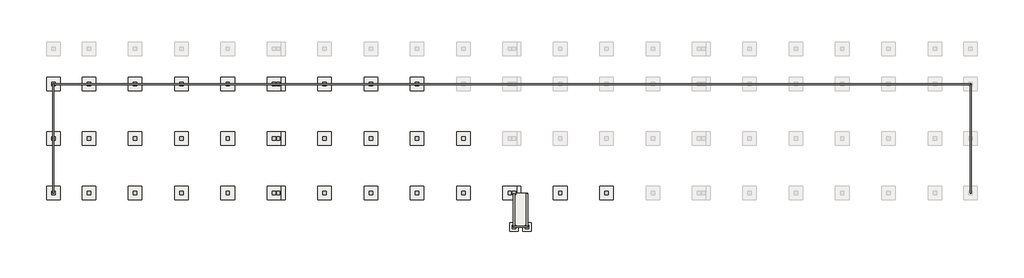
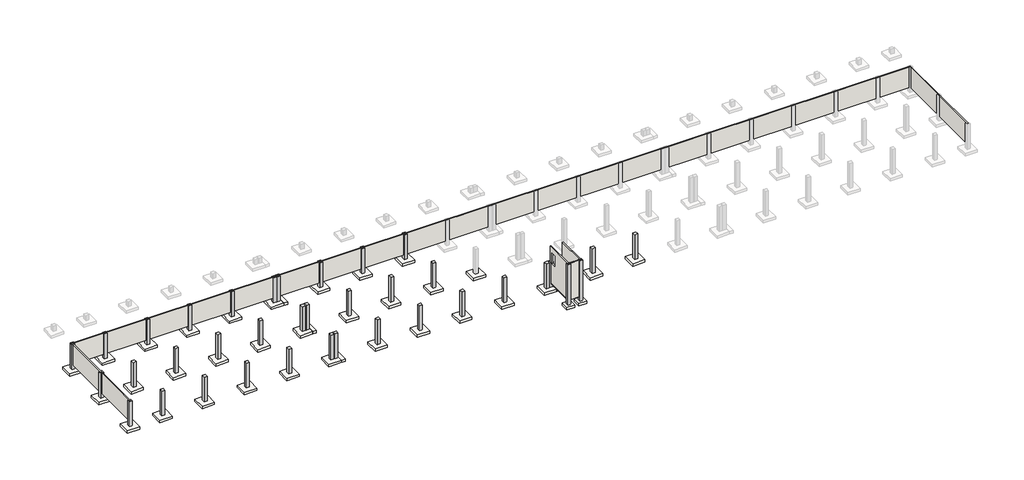
# Not in any storey, part 1 of 3: 39 slabs, 37 columns, 6 walls.
"""IFC4 building model written with IfcOpenShell, lengths in millimetres."""

import ifcopenshell
import ifcopenshell.guid

model = None  # the IFC model being written
_history = None  # IfcOwnerHistory: only IFC2X3 demands one
_inside = {}  # id of a spatial element -> (the spatial element, [elements in it])
_under = {}  # id of a project, library or spatial element -> (it, [spatial elements below it])
_declared = {}  # id of a project -> (the project, [libraries it declares])
_typed = {}  # id of a type object -> (the type object, [elements of that type])
_made_of = {}  # id of a material, layer set ... -> (it, [elements and type objects made of it])


def new_model(schema):
    """Start an empty IFC model of exactly this schema.

    Asked for "IFC4X3", IfcOpenShell would pick the latest addendum, in which some entities
    have other attributes; the version numbers below select the first issue.
    IFC2X3 requires an IfcOwnerHistory on every rooted entity: one is made here for all.
    """
    global model, _history
    if schema == "IFC4X3":
        model = ifcopenshell.file(schema_version=(4, 3, 0, 0))
    else:
        model = ifcopenshell.file(schema=schema)
    _inside.clear()
    _under.clear()
    _declared.clear()
    _typed.clear()
    _made_of.clear()
    _history = None
    if model.schema == "IFC2X3":
        org = make("IfcOrganization", Name="unknown")
        user = make(
            "IfcPersonAndOrganization",
            ThePerson=make("IfcPerson", FamilyName="unknown"),
            TheOrganization=org,
        )
        app = make(
            "IfcApplication",
            ApplicationDeveloper=org,
            Version="unknown",
            ApplicationFullName="unknown",
            ApplicationIdentifier="unknown",
        )
        _history = make(
            "IfcOwnerHistory",
            OwningUser=user,
            OwningApplication=app,
            ChangeAction="ADDED",
            CreationDate=0,
        )
    return model


def make(cls, **values):
    """One entity of the class cls with the attributes given. An attribute that is None is left unset."""
    return model.create_entity(
        cls, **{name: value for name, value in values.items() if value is not None}
    )


def rooted(cls, **values):
    """An entity with a GlobalId (a new one), such as an element, a storey or a relation."""
    return make(cls, GlobalId=ifcopenshell.guid.new(), OwnerHistory=_history, **values)


def si_unit(unit_type, name, prefix=None):
    """IfcSIUnit, for example si_unit("LENGTHUNIT", "METRE", prefix="MILLI")."""
    return make("IfcSIUnit", UnitType=unit_type, Prefix=prefix, Name=name)


def assignment(units):
    """IfcUnitAssignment: the units of a project."""
    return None if units is None else make("IfcUnitAssignment", Units=units)


def point(xyz):
    """IfcCartesianPoint."""
    return None if xyz is None else make("IfcCartesianPoint", Coordinates=xyz)


def direction(xyz):
    """IfcDirection."""
    return None if xyz is None else make("IfcDirection", DirectionRatios=xyz)


def frame(location, z_axis=None, x_axis=None):
    """IfcAxis2Placement3D, a coordinate frame: its origin and axes. An axis left out is left unset."""
    return make(
        "IfcAxis2Placement3D",
        Location=point(location),
        Axis=direction(z_axis),
        RefDirection=direction(x_axis),
    )


def origin():
    """The frame at (0, 0, 0) with its axes left unset."""
    return frame((0.0, 0.0, 0.0))


def place(relative_to, where):
    """IfcLocalPlacement: puts the frame where relative to a parent placement (None: the world)."""
    return make(
        "IfcLocalPlacement", PlacementRelTo=relative_to, RelativePlacement=where
    )


def context(
    kind, dimensions, precision=None, world=None, true_north=None, identifier=None
):
    """IfcGeometricRepresentationContext, for example the 3D "Model" context."""
    return make(
        "IfcGeometricRepresentationContext",
        ContextIdentifier=identifier,
        ContextType=kind,
        CoordinateSpaceDimension=dimensions,
        Precision=precision,
        WorldCoordinateSystem=world,
        TrueNorth=true_north,
    )


def project(units=None, contexts=None):
    """IfcProject with its units and contexts."""
    return rooted(
        "IfcProject",
        Name="project",
        RepresentationContexts=contexts,
        UnitsInContext=assignment(units),
    )


def spatial(cls, under=None, at=None, **own):
    """A site, building, storey or space (cls), placed at a placement, below another one or the project."""
    s = rooted(cls, ObjectPlacement=at, **own)
    if under is not None:
        _under.setdefault(under.id(), (under, []))[1].append(s)
    return s


def polyline(points):
    """IfcPolyline through the points."""
    return make("IfcPolyline", Points=[point(p) for p in points])


def outline(outer, holes=None, kind="AREA"):
    """IfcArbitraryClosedProfileDef: a profile drawn as a closed curve; with holes, ...WithVoids."""
    if holes is None:
        return make("IfcArbitraryClosedProfileDef", ProfileType=kind, OuterCurve=outer)
    return make(
        "IfcArbitraryProfileDefWithVoids",
        ProfileType=kind,
        OuterCurve=outer,
        InnerCurves=holes,
    )


def extrude(swept, where, along, depth):
    """IfcExtrudedAreaSolid: the profile swept, set in the frame where, extruded along a direction by depth."""
    return make(
        "IfcExtrudedAreaSolid",
        SweptArea=swept,
        Position=where,
        ExtrudedDirection=direction(along),
        Depth=depth,
    )


def faces_of(points, faces, orient=None, outer=None):
    """IfcFace entities. A face is a list of loops; a loop is a list of indices into points, from 0.

    orient and outer hold one flag for each loop. By default every Orientation is true, the
    first loop of a face is its IfcFaceOuterBound and the others are IfcFaceBound.
    """
    made = []
    for i, loops in enumerate(faces):
        bounds = []
        for j, loop in enumerate(loops):
            is_outer = j == 0 if outer is None else outer[i][j]
            bounds.append(
                make(
                    "IfcFaceOuterBound" if is_outer else "IfcFaceBound",
                    Bound=make("IfcPolyLoop", Polygon=[points[k] for k in loop]),
                    Orientation=True if orient is None else orient[i][j],
                )
            )
        made.append(make("IfcFace", Bounds=bounds))
    return made


def faceted_brep(points, faces, orient=None, outer=None, voids=None):
    """IfcFacetedBrep: a solid bounded by flat faces; with voids (closed shells), ...WithVoids."""
    shared = [point(p) for p in points]
    hull = make("IfcClosedShell", CfsFaces=faces_of(shared, faces, orient, outer))
    if voids is None:
        return make("IfcFacetedBrep", Outer=hull)
    return make(
        "IfcFacetedBrepWithVoids",
        Outer=hull,
        Voids=[
            make(cls, CfsFaces=faces_of(shared, fs, o, b)) for cls, fs, o, b in voids
        ],
    )


def shape(context_of_items, identifier, shape_type, items):
    """IfcShapeRepresentation: the items that make up one representation, for example the "Body"."""
    return make(
        "IfcShapeRepresentation",
        ContextOfItems=context_of_items,
        RepresentationIdentifier=identifier,
        RepresentationType=shape_type,
        Items=items,
    )


def source(mapping_origin, context_of_items, identifier, shape_type, items):
    """IfcRepresentationMap: a shape defined once, which mapped items show again and again."""
    return make(
        "IfcRepresentationMap",
        MappingOrigin=mapping_origin,
        MappedRepresentation=shape(context_of_items, identifier, shape_type, items),
    )


def transform(
    local_origin,
    x_axis=None,
    y_axis=None,
    z_axis=None,
    scale=None,
    scale2=None,
    scale3=None,
    uniform=True,
):
    """IfcCartesianTransformationOperator3D, or its non-uniform kind. x_axis, y_axis, z_axis: its Axis1, 2, 3."""
    if uniform:
        return make(
            "IfcCartesianTransformationOperator3D",
            Axis1=direction(x_axis),
            Axis2=direction(y_axis),
            LocalOrigin=point(local_origin),
            Scale=scale,
            Axis3=direction(z_axis),
        )
    return make(
        "IfcCartesianTransformationOperator3DnonUniform",
        Axis1=direction(x_axis),
        Axis2=direction(y_axis),
        LocalOrigin=point(local_origin),
        Scale=scale,
        Axis3=direction(z_axis),
        Scale2=scale2,
        Scale3=scale3,
    )


def mapped(mapping_source, mapping_target):
    """IfcMappedItem: shows the shape of a source again, moved by a transform."""
    return make(
        "IfcMappedItem", MappingSource=mapping_source, MappingTarget=mapping_target
    )


def made_of(thing, what):
    """Note that an element or type object is made of a material, layer set ...; save() writes the relation."""
    if what is not None:
        _made_of.setdefault(what.id(), (what, []))[1].append(thing)
    return thing


def element(
    cls,
    number,
    at=None,
    inside=None,
    cuts=None,
    type_object=None,
    material=None,
    context=None,
    identifier="Body",
    shape_type=None,
    held_by="IfcProductDefinitionShape",
    body=None,
    shapes=None,
    **own,
):
    """One element of the class cls, such as IfcWall. Its Tag is "e" and its number.

    at: its placement. inside: the storey or other place that contains it. cuts: it is an
    opening in that element (IfcRelVoidsElement). A single representation is given by context,
    identifier, shape_type and body (its items); several are given by shapes. held_by: the class
    of the entity that holds the representations. save() writes the other relations.
    """
    e = rooted(cls, Tag="e%d" % number, ObjectPlacement=at, **own)
    if body is not None:
        shapes = [shape(context, identifier, shape_type, body)]
    if shapes is not None:
        e.Representation = make(held_by, Representations=shapes)
    if inside is not None:
        _inside.setdefault(inside.id(), (inside, []))[1].append(e)
    if cuts is not None:
        rooted(
            "IfcRelVoidsElement", RelatingBuildingElement=cuts, RelatedOpeningElement=e
        )
    if type_object is not None:
        _typed.setdefault(type_object.id(), (type_object, []))[1].append(e)
    return made_of(e, material)


def aggregate(whole, parts):
    """IfcRelAggregates: a whole, such as a stair, and the parts it consists of."""
    return rooted("IfcRelAggregates", RelatingObject=whole, RelatedObjects=parts)


def save(model, path):
    """Write the relations noted so far, then the file.

    IfcRelAggregates (storeys below a building ...), IfcRelContainedInSpatialStructure (elements
    in a storey), IfcRelDefinesByType, IfcRelAssociatesMaterial and IfcRelDeclares: one each for
    every whole, place, type object, material and project.
    """
    for whole, parts in _under.values():
        aggregate(whole, parts)
    for where, things in _inside.values():
        rooted(
            "IfcRelContainedInSpatialStructure",
            RelatedElements=things,
            RelatingStructure=where,
        )
    for kind, things in _typed.values():
        rooted("IfcRelDefinesByType", RelatedObjects=things, RelatingType=kind)
    for what, things in _made_of.values():
        rooted("IfcRelAssociatesMaterial", RelatedObjects=things, RelatingMaterial=what)
    for by, libraries in _declared.values():
        rooted("IfcRelDeclares", RelatingContext=by, RelatedDefinitions=libraries)
    model.write(path)


def foundation_rectangular_non_pile_5fe39465(model_context):
    return source(origin(), model_context, "Body", "SweptSolid", [
        extrude(outline(polyline([(1200.0, 1200.0), (1200.0, -1200.0), (-1200.0, -1200.0), (-1200.0, 1200.0), (1200.0, 1200.0)])), frame((0.0, 0.0, -500.0), z_axis=(0.0, 0.0, 1.0), x_axis=(1.0, 0.0, 0.0)), (0.0, 0.0, 1.0), 500.0),
    ])


model = new_model("IFC4")

# Units and contexts
model_context = context("Model", 3, world=origin())
ifc_project = project(units=[si_unit("LENGTHUNIT", "METRE", prefix="MILLI")], contexts=[model_context])

# Site, building
site = spatial("IfcSite", under=ifc_project)
building = spatial("IfcBuilding", under=site)

# Columns
placement = place(None, origin())
element("IfcColumn", 1, ObjectType="RC_Column_Rectangular : H_SC_AR_S15_UG PED_W600xL600_Bit_Anchor", at=placement, inside=building, context=model_context, shape_type="SweptSolid", body=[
    extrude(outline(polyline([(-4070.0, -5700.4791411), (-4070.0, -6300.4791411), (-4670.0, -6300.4791411), (-4670.0, -5700.4791411), (-4070.0, -5700.4791411)])), frame((0.0, 0.0, -4800.0381366), z_axis=(0.0, 0.0, 1.0), x_axis=(1.0, 0.0, 0.0)), (0.0, 0.0, 1.0), 5100.0),
])
element("IfcColumn", 2, ObjectType="RC_Column_Rectangular : H_SC_AR_S15_UG PED_W600xL600_Bit_Anchor", at=placement, inside=building, context=model_context, shape_type="SweptSolid", body=[
    extrude(outline(polyline([(2230.0, -5700.4791411), (2230.0, -6300.4791411), (1630.0, -6300.4791411), (1630.0, -5700.4791411), (2230.0, -5700.4791411)])), frame((0.0, 0.0, -4800.0381366), z_axis=(0.0, 0.0, 1.0), x_axis=(1.0, 0.0, 0.0)), (0.0, 0.0, 1.0), 5100.0),
])
element("IfcColumn", 3, ObjectType="RC_Column_Rectangular : H_SC_AR_S15_UG PED_W600xL600_Bit_Anchor", at=placement, inside=building, context=model_context, shape_type="SweptSolid", body=[
    extrude(outline(polyline([(10430.0, -5700.4791411), (10430.0, -6300.4791411), (9830.0, -6300.4791411), (9830.0, -5700.4791411), (10430.0, -5700.4791411)])), frame((0.0, 0.0, -4800.0381366), z_axis=(0.0, 0.0, 1.0), x_axis=(1.0, 0.0, 0.0)), (0.0, 0.0, 1.0), 5100.0),
])
element("IfcColumn", 4, ObjectType="RC_Column_Rectangular : H_SC_AR_S15_UG PED_W600xL600_Bit_Anchor", at=placement, inside=building, context=model_context, shape_type="SweptSolid", body=[
    extrude(outline(polyline([(18630.0, -5700.4791411), (18630.0, -6300.4791411), (18030.0, -6300.4791411), (18030.0, -5700.4791411), (18630.0, -5700.4791411)])), frame((0.0, 0.0, -4800.0381366), z_axis=(0.0, 0.0, 1.0), x_axis=(1.0, 0.0, 0.0)), (0.0, 0.0, 1.0), 5100.0),
])
element("IfcColumn", 5, ObjectType="RC_Column_Rectangular : H_SC_AR_S15_UG PED_W600xL600_Bit_Anchor", at=placement, inside=building, context=model_context, shape_type="SweptSolid", body=[
    extrude(outline(polyline([(26830.0, -5700.4791411), (26830.0, -6300.4791411), (26230.0, -6300.4791411), (26230.0, -5700.4791411), (26830.0, -5700.4791411)])), frame((0.0, 0.0, -4800.0381366), z_axis=(0.0, 0.0, 1.0), x_axis=(1.0, 0.0, 0.0)), (0.0, 0.0, 1.0), 5100.0),
])
element("IfcColumn", 6, ObjectType="RC_Column_Rectangular : H_SC_AR_S15_UG PED_W600xL600_Bit_Anchor", at=placement, inside=building, context=model_context, shape_type="SweptSolid", body=[
    extrude(outline(polyline([(35030.0, -5700.4791411), (35030.0, -6300.4791411), (34430.0, -6300.4791411), (34430.0, -5700.4791411), (35030.0, -5700.4791411)])), frame((0.0, 0.0, -4800.0381366), z_axis=(0.0, 0.0, 1.0), x_axis=(1.0, 0.0, 0.0)), (0.0, 0.0, 1.0), 5100.0),
])
element("IfcColumn", 7, ObjectType="RC_Column_Rectangular : H_SC_AR_S15_UG PED_W600xL600_Bit_Anchor", at=placement, inside=building, context=model_context, shape_type="SweptSolid", body=[
    extrude(outline(polyline([(35780.0, -5700.4791411), (35780.0, -6300.4791411), (35180.0, -6300.4791411), (35180.0, -5700.4791411), (35780.0, -5700.4791411)])), frame((0.0, 0.0, -4800.0381366), z_axis=(0.0, 0.0, 1.0), x_axis=(1.0, 0.0, 0.0)), (0.0, 0.0, 1.0), 5100.0),
])
element("IfcColumn", 8, ObjectType="RC_Column_Rectangular : H_SC_AR_S15_UG PED_W600xL600_Bit_Anchor", at=placement, inside=building, context=model_context, shape_type="SweptSolid", body=[
    extrude(outline(polyline([(43980.0, -5700.4791411), (43980.0, -6300.4791411), (43380.0, -6300.4791411), (43380.0, -5700.4791411), (43980.0, -5700.4791411)])), frame((0.0, 0.0, -4800.0381366), z_axis=(0.0, 0.0, 1.0), x_axis=(1.0, 0.0, 0.0)), (0.0, 0.0, 1.0), 5100.0),
])
element("IfcColumn", 9, ObjectType="RC_Column_Rectangular : H_SC_AR_S15_UG PED_W600xL600_Bit_Anchor", at=placement, inside=building, context=model_context, shape_type="SweptSolid", body=[
    extrude(outline(polyline([(52180.0, -5700.4791411), (52180.0, -6300.4791411), (51580.0, -6300.4791411), (51580.0, -5700.4791411), (52180.0, -5700.4791411)])), frame((0.0, 0.0, -4800.0381366), z_axis=(0.0, 0.0, 1.0), x_axis=(1.0, 0.0, 0.0)), (0.0, 0.0, 1.0), 5100.0),
])
element("IfcColumn", 10, ObjectType="RC_Column_Rectangular : H_SC_AR_S15_UG PED_W600xL600_Bit_Anchor", at=placement, inside=building, context=model_context, shape_type="SweptSolid", body=[
    extrude(outline(polyline([(60380.0, -5700.4791411), (60380.0, -6300.4791411), (59780.0, -6300.4791411), (59780.0, -5700.4791411), (60380.0, -5700.4791411)])), frame((0.0, 0.0, -4800.0381366), z_axis=(0.0, 0.0, 1.0), x_axis=(1.0, 0.0, 0.0)), (0.0, 0.0, 1.0), 5100.0),
])
element("IfcColumn", 11, ObjectType="RC_Column_Rectangular : H_SC_AR_S15_UG PED_W600xL600_Bit_Anchor", at=placement, inside=building, context=model_context, shape_type="SweptSolid", body=[
    extrude(outline(polyline([(-4070.0, -15350.4791411), (-4070.0, -15950.4791411), (-4670.0, -15950.4791411), (-4670.0, -15350.4791411), (-4070.0, -15350.4791411)])), frame((0.0, 0.0, -4800.0381366), z_axis=(0.0, 0.0, 1.0), x_axis=(1.0, 0.0, 0.0)), (0.0, 0.0, 1.0), 5100.0),
])
element("IfcColumn", 12, ObjectType="RC_Column_Rectangular : H_SC_AR_S15_UG PED_W600xL600_Bit_Anchor", at=placement, inside=building, context=model_context, shape_type="SweptSolid", body=[
    extrude(outline(polyline([(2230.0, -15350.4791411), (2230.0, -15950.4791411), (1630.0, -15950.4791411), (1630.0, -15350.4791411), (2230.0, -15350.4791411)])), frame((0.0, 0.0, -4800.0381366), z_axis=(0.0, 0.0, 1.0), x_axis=(1.0, 0.0, 0.0)), (0.0, 0.0, 1.0), 5100.0),
])
element("IfcColumn", 13, ObjectType="RC_Column_Rectangular : H_SC_AR_S15_UG PED_W600xL600_Bit_Anchor", at=placement, inside=building, context=model_context, shape_type="SweptSolid", body=[
    extrude(outline(polyline([(10430.0, -15350.4791411), (10430.0, -15950.4791411), (9830.0, -15950.4791411), (9830.0, -15350.4791411), (10430.0, -15350.4791411)])), frame((0.0, 0.0, -4800.0381366), z_axis=(0.0, 0.0, 1.0), x_axis=(1.0, 0.0, 0.0)), (0.0, 0.0, 1.0), 5100.0),
])
element("IfcColumn", 14, ObjectType="RC_Column_Rectangular : H_SC_AR_S15_UG PED_W600xL600_Bit_Anchor", at=placement, inside=building, context=model_context, shape_type="SweptSolid", body=[
    extrude(outline(polyline([(18630.0, -15350.4791411), (18630.0, -15950.4791411), (18030.0, -15950.4791411), (18030.0, -15350.4791411), (18630.0, -15350.4791411)])), frame((0.0, 0.0, -4800.0381366), z_axis=(0.0, 0.0, 1.0), x_axis=(1.0, 0.0, 0.0)), (0.0, 0.0, 1.0), 5100.0),
])
element("IfcColumn", 15, ObjectType="RC_Column_Rectangular : H_SC_AR_S15_UG PED_W600xL600_Bit_Anchor", at=placement, inside=building, context=model_context, shape_type="SweptSolid", body=[
    extrude(outline(polyline([(26830.0, -15350.4791411), (26830.0, -15950.4791411), (26230.0, -15950.4791411), (26230.0, -15350.4791411), (26830.0, -15350.4791411)])), frame((0.0, 0.0, -4800.0381366), z_axis=(0.0, 0.0, 1.0), x_axis=(1.0, 0.0, 0.0)), (0.0, 0.0, 1.0), 5100.0),
])
element("IfcColumn", 16, ObjectType="RC_Column_Rectangular : H_SC_AR_S15_UG PED_W600xL600_Bit_Anchor", at=placement, inside=building, context=model_context, shape_type="SweptSolid", body=[
    extrude(outline(polyline([(35030.0, -15350.4791411), (35030.0, -15950.4791411), (34430.0, -15950.4791411), (34430.0, -15350.4791411), (35030.0, -15350.4791411)])), frame((0.0, 0.0, -4800.0381366), z_axis=(0.0, 0.0, 1.0), x_axis=(1.0, 0.0, 0.0)), (0.0, 0.0, 1.0), 5100.0),
])
element("IfcColumn", 17, ObjectType="RC_Column_Rectangular : H_SC_AR_S15_UG PED_W600xL600_Bit_Anchor", at=placement, inside=building, context=model_context, shape_type="SweptSolid", body=[
    extrude(outline(polyline([(35780.0, -15350.4791411), (35780.0, -15950.4791411), (35180.0, -15950.4791411), (35180.0, -15350.4791411), (35780.0, -15350.4791411)])), frame((0.0, 0.0, -4800.0381366), z_axis=(0.0, 0.0, 1.0), x_axis=(1.0, 0.0, 0.0)), (0.0, 0.0, 1.0), 5100.0),
])
element("IfcColumn", 18, ObjectType="RC_Column_Rectangular : H_SC_AR_S15_UG PED_W600xL600_Bit_Anchor", at=placement, inside=building, context=model_context, shape_type="SweptSolid", body=[
    extrude(outline(polyline([(43980.0, -15350.4791411), (43980.0, -15950.4791411), (43380.0, -15950.4791411), (43380.0, -15350.4791411), (43980.0, -15350.4791411)])), frame((0.0, 0.0, -4800.0381366), z_axis=(0.0, 0.0, 1.0), x_axis=(1.0, 0.0, 0.0)), (0.0, 0.0, 1.0), 5100.0),
])
element("IfcColumn", 19, ObjectType="RC_Column_Rectangular : H_SC_AR_S15_UG PED_W600xL600_Bit_Anchor", at=placement, inside=building, context=model_context, shape_type="SweptSolid", body=[
    extrude(outline(polyline([(52180.0, -15350.4791411), (52180.0, -15950.4791411), (51580.0, -15950.4791411), (51580.0, -15350.4791411), (52180.0, -15350.4791411)])), frame((0.0, 0.0, -4800.0381366), z_axis=(0.0, 0.0, 1.0), x_axis=(1.0, 0.0, 0.0)), (0.0, 0.0, 1.0), 5100.0),
])
element("IfcColumn", 20, ObjectType="RC_Column_Rectangular : H_SC_AR_S15_UG PED_W600xL600_Bit_Anchor", at=placement, inside=building, context=model_context, shape_type="SweptSolid", body=[
    extrude(outline(polyline([(60380.0, -15350.4791411), (60380.0, -15950.4791411), (59780.0, -15950.4791411), (59780.0, -15350.4791411), (60380.0, -15350.4791411)])), frame((0.0, 0.0, -4800.0381366), z_axis=(0.0, 0.0, 1.0), x_axis=(1.0, 0.0, 0.0)), (0.0, 0.0, 1.0), 5100.0),
])
element("IfcColumn", 21, ObjectType="RC_Column_Rectangular : H_SC_AR_S15_UG PED_W600xL600_Bit_Anchor", at=placement, inside=building, context=model_context, shape_type="SweptSolid", body=[
    extrude(outline(polyline([(-4070.0, -25000.4791411), (-4070.0, -25600.4791411), (-4670.0, -25600.4791411), (-4670.0, -25000.4791411), (-4070.0, -25000.4791411)])), frame((0.0, 0.0, -4800.0381366), z_axis=(0.0, 0.0, 1.0), x_axis=(1.0, 0.0, 0.0)), (0.0, 0.0, 1.0), 5100.0),
])
element("IfcColumn", 22, ObjectType="RC_Column_Rectangular : H_SC_AR_S15_UG PED_W600xL600_Bit_Anchor", at=placement, inside=building, context=model_context, shape_type="SweptSolid", body=[
    extrude(outline(polyline([(2230.0, -25000.4791411), (2230.0, -25600.4791411), (1630.0, -25600.4791411), (1630.0, -25000.4791411), (2230.0, -25000.4791411)])), frame((0.0, 0.0, -4800.0381366), z_axis=(0.0, 0.0, 1.0), x_axis=(1.0, 0.0, 0.0)), (0.0, 0.0, 1.0), 5100.0),
])
element("IfcColumn", 23, ObjectType="RC_Column_Rectangular : H_SC_AR_S15_UG PED_W600xL600_Bit_Anchor", at=placement, inside=building, context=model_context, shape_type="SweptSolid", body=[
    extrude(outline(polyline([(10430.0, -25000.4791411), (10430.0, -25600.4791411), (9830.0, -25600.4791411), (9830.0, -25000.4791411), (10430.0, -25000.4791411)])), frame((0.0, 0.0, -4800.0381366), z_axis=(0.0, 0.0, 1.0), x_axis=(1.0, 0.0, 0.0)), (0.0, 0.0, 1.0), 5100.0),
])
element("IfcColumn", 24, ObjectType="RC_Column_Rectangular : H_SC_AR_S15_UG PED_W600xL600_Bit_Anchor", at=placement, inside=building, context=model_context, shape_type="SweptSolid", body=[
    extrude(outline(polyline([(18630.0, -25000.4791411), (18630.0, -25600.4791411), (18030.0, -25600.4791411), (18030.0, -25000.4791411), (18630.0, -25000.4791411)])), frame((0.0, 0.0, -4800.0381366), z_axis=(0.0, 0.0, 1.0), x_axis=(1.0, 0.0, 0.0)), (0.0, 0.0, 1.0), 5100.0),
])
element("IfcColumn", 25, ObjectType="RC_Column_Rectangular : H_SC_AR_S15_UG PED_W600xL600_Bit_Anchor", at=placement, inside=building, context=model_context, shape_type="SweptSolid", body=[
    extrude(outline(polyline([(26830.0, -25000.4791411), (26830.0, -25600.4791411), (26230.0, -25600.4791411), (26230.0, -25000.4791411), (26830.0, -25000.4791411)])), frame((0.0, 0.0, -4800.0381366), z_axis=(0.0, 0.0, 1.0), x_axis=(1.0, 0.0, 0.0)), (0.0, 0.0, 1.0), 5100.0),
])
element("IfcColumn", 26, ObjectType="RC_Column_Rectangular : H_SC_AR_S15_UG PED_W600xL600_Bit_Anchor", at=placement, inside=building, context=model_context, shape_type="SweptSolid", body=[
    extrude(outline(polyline([(35030.0, -25000.4791411), (35030.0, -25600.4791411), (34430.0, -25600.4791411), (34430.0, -25000.4791411), (35030.0, -25000.4791411)])), frame((0.0, 0.0, -4800.0381366), z_axis=(0.0, 0.0, 1.0), x_axis=(1.0, 0.0, 0.0)), (0.0, 0.0, 1.0), 5100.0),
])
element("IfcColumn", 27, ObjectType="RC_Column_Rectangular : H_SC_AR_S15_UG PED_W600xL600_Bit_Anchor", at=placement, inside=building, context=model_context, shape_type="SweptSolid", body=[
    extrude(outline(polyline([(35780.0, -25000.4791411), (35780.0, -25600.4791411), (35180.0, -25600.4791411), (35180.0, -25000.4791411), (35780.0, -25000.4791411)])), frame((0.0, 0.0, -4800.0381366), z_axis=(0.0, 0.0, 1.0), x_axis=(1.0, 0.0, 0.0)), (0.0, 0.0, 1.0), 5100.0),
])
element("IfcColumn", 28, ObjectType="RC_Column_Rectangular : H_SC_AR_S15_UG PED_W600xL600_Bit_Anchor", at=placement, inside=building, context=model_context, shape_type="SweptSolid", body=[
    extrude(outline(polyline([(43980.0, -25000.4791411), (43980.0, -25600.4791411), (43380.0, -25600.4791411), (43380.0, -25000.4791411), (43980.0, -25000.4791411)])), frame((0.0, 0.0, -4800.0381366), z_axis=(0.0, 0.0, 1.0), x_axis=(1.0, 0.0, 0.0)), (0.0, 0.0, 1.0), 5100.0),
])
element("IfcColumn", 29, ObjectType="RC_Column_Rectangular : H_SC_AR_S15_UG PED_W600xL600_Bit_Anchor", at=placement, inside=building, context=model_context, shape_type="SweptSolid", body=[
    extrude(outline(polyline([(52180.0, -25000.4791411), (52180.0, -25600.4791411), (51580.0, -25600.4791411), (51580.0, -25000.4791411), (52180.0, -25000.4791411)])), frame((0.0, 0.0, -4800.0381366), z_axis=(0.0, 0.0, 1.0), x_axis=(1.0, 0.0, 0.0)), (0.0, 0.0, 1.0), 5100.0),
])
element("IfcColumn", 30, ObjectType="RC_Column_Rectangular : H_SC_AR_S15_UG PED_W600xL600_Bit_Anchor", at=placement, inside=building, context=model_context, shape_type="SweptSolid", body=[
    extrude(outline(polyline([(60380.0, -25000.4791411), (60380.0, -25600.4791411), (59780.0, -25600.4791411), (59780.0, -25000.4791411), (60380.0, -25000.4791411)])), frame((0.0, 0.0, -4800.0381366), z_axis=(0.0, 0.0, 1.0), x_axis=(1.0, 0.0, 0.0)), (0.0, 0.0, 1.0), 5100.0),
])
element("IfcColumn", 31, ObjectType="RC_Column_Rectangular : H_SC_AR_S15_UG PED_W600xL600_Bit_Anchor", at=placement, inside=building, context=model_context, shape_type="SweptSolid", body=[
    extrude(outline(polyline([(68580.0, -25000.4791411), (68580.0, -25600.4791411), (67980.0, -25600.4791411), (67980.0, -25000.4791411), (68580.0, -25000.4791411)])), frame((0.0, 0.0, -4800.0381366), z_axis=(0.0, 0.0, 1.0), x_axis=(1.0, 0.0, 0.0)), (0.0, 0.0, 1.0), 5100.0),
])
element("IfcColumn", 32, ObjectType="RC_Column_Rectangular : H_SC_AR_S15_UG PED_W600xL600_Bit_Anchor", at=placement, inside=building, context=model_context, shape_type="SweptSolid", body=[
    extrude(outline(polyline([(76780.0, -25000.4791411), (76780.0, -25600.4791411), (76180.0, -25600.4791411), (76180.0, -25000.4791411), (76780.0, -25000.4791411)])), frame((0.0, 0.0, -4800.0381366), z_axis=(0.0, 0.0, 1.0), x_axis=(1.0, 0.0, 0.0)), (0.0, 0.0, 1.0), 5100.0),
])
element("IfcColumn", 33, ObjectType="RC_Column_Rectangular : H_SC_AR_S15_UG PED_W600xL600_Bit_Anchor", at=placement, inside=building, context=model_context, shape_type="SweptSolid", body=[
    extrude(outline(polyline([(77530.0, -25000.4791411), (77530.0, -25600.4791411), (76930.0, -25600.4791411), (76930.0, -25000.4791411), (77530.0, -25000.4791411)])), frame((0.0, 0.0, -4800.0381366), z_axis=(0.0, 0.0, 1.0), x_axis=(1.0, 0.0, 0.0)), (0.0, 0.0, 1.0), 5100.0),
])
element("IfcColumn", 34, ObjectType="RC_Column_Rectangular : H_SC_AR_S15_UG PED_W600xL600_Bit_Anchor", at=placement, inside=building, context=model_context, shape_type="SweptSolid", body=[
    extrude(outline(polyline([(85730.0, -25000.4791411), (85730.0, -25600.4791411), (85130.0, -25600.4791411), (85130.0, -25000.4791411), (85730.0, -25000.4791411)])), frame((0.0, 0.0, -4800.0381366), z_axis=(0.0, 0.0, 1.0), x_axis=(1.0, 0.0, 0.0)), (0.0, 0.0, 1.0), 5100.0),
])
element("IfcColumn", 35, ObjectType="RC_Column_Rectangular : H_SC_AR_S15_UG PED_W600xL600_Bit_Anchor", at=placement, inside=building, context=model_context, shape_type="SweptSolid", body=[
    extrude(outline(polyline([(93930.0, -25000.4791411), (93930.0, -25600.4791411), (93330.0, -25600.4791411), (93330.0, -25000.4791411), (93930.0, -25000.4791411)])), frame((0.0, 0.0, -4800.0381366), z_axis=(0.0, 0.0, 1.0), x_axis=(1.0, 0.0, 0.0)), (0.0, 0.0, 1.0), 5100.0),
])
element("IfcColumn", 36, ObjectType="RC_Column_Rectangular : H_SC_AR_S15_UG PED_W600xL600_Bit_Anchor", at=placement, inside=building, context=model_context, shape_type="SweptSolid", body=[
    extrude(outline(polyline([(77530.0, -31000.4791411), (77530.0, -31600.4791411), (76930.0, -31600.4791411), (76930.0, -31000.4791411), (77530.0, -31000.4791411)])), frame((0.0, 0.0, -4800.0381366), z_axis=(0.0, 0.0, 1.0), x_axis=(1.0, 0.0, 0.0)), (0.0, 0.0, 1.0), 8250.0),
])
element("IfcColumn", 37, ObjectType="RC_Column_Rectangular : H_SC_AR_S15_UG PED_W600xL600_Bit_Anchor", at=placement, inside=building, context=model_context, shape_type="SweptSolid", body=[
    extrude(outline(polyline([(79847.0, -31000.4791411), (79847.0, -31600.4791411), (79247.0, -31600.4791411), (79247.0, -31000.4791411), (79847.0, -31000.4791411)])), frame((0.0, 0.0, -4800.0381366), z_axis=(0.0, 0.0, 1.0), x_axis=(1.0, 0.0, 0.0)), (0.0, 0.0, 1.0), 8250.0),
])

# Slabs
element("IfcSlab", 38, ObjectType="H_FL_AR_S17_RC Slab T150", at=placement, inside=building, context=model_context, shape_type="SweptSolid", body=[
    extrude(outline(polyline([(79642.0, -25300.4791411), (79642.0, -31300.4791411), (77130.0, -31300.4791411), (77130.0, -25300.4791411), (79642.0, -25300.4791411)])), frame((0.0, 0.0, -4100.0381366), z_axis=(0.0, 0.0, 1.0), x_axis=(1.0, 0.0, 0.0)), (0.0, 0.0, 1.0), 150.0),
])
element("IfcSlab", 39, ObjectType="Foundation Rectangular (Non-Pile) : H_SF_AR_S18_W2400xL2400xT500_Bitumen", at=placement, inside=building, context=model_context, shape_type="SweptSolid", body=[
    extrude(outline(polyline([(35930.0, -4800.4791411), (35930.0, -7200.4791411), (33530.0, -7200.4791411), (33530.0, -4800.4791411), (35930.0, -4800.4791411)])), frame((0.0, 0.0, -5300.0381366), z_axis=(0.0, 0.0, 1.0), x_axis=(1.0, 0.0, 0.0)), (0.0, 0.0, 1.0), 500.0),
])
element("IfcSlab", 40, ObjectType="Foundation Rectangular (Non-Pile) : H_SF_AR_S18_W2400xL2400xT500_Bitumen", at=placement, inside=building, context=model_context, shape_type="SweptSolid", body=[
    extrude(outline(polyline([(36680.0, -4800.4791411), (36680.0, -7200.4791411), (35930.0, -7200.4791411), (35930.0, -4800.4791411), (36680.0, -4800.4791411)])), frame((0.0, 0.0, -5300.0381366), z_axis=(0.0, 0.0, 1.0), x_axis=(1.0, 0.0, 0.0)), (0.0, 0.0, 1.0), 500.0),
])
element("IfcSlab", 41, ObjectType="Foundation Rectangular (Non-Pile) : H_SF_AR_S18_W2400xL2400xT500_Bitumen", at=placement, inside=building, context=model_context, shape_type="SweptSolid", body=[
    extrude(outline(polyline([(35930.0, -14450.4791411), (35930.0, -16850.4791411), (33530.0, -16850.4791411), (33530.0, -14450.4791411), (35930.0, -14450.4791411)])), frame((0.0, 0.0, -5300.0381366), z_axis=(0.0, 0.0, 1.0), x_axis=(1.0, 0.0, 0.0)), (0.0, 0.0, 1.0), 500.0),
])
element("IfcSlab", 42, ObjectType="Foundation Rectangular (Non-Pile) : H_SF_AR_S18_W2400xL2400xT500_Bitumen", at=placement, inside=building, context=model_context, shape_type="SweptSolid", body=[
    extrude(outline(polyline([(36680.0, -14450.4791411), (36680.0, -16850.4791411), (35930.0, -16850.4791411), (35930.0, -14450.4791411), (36680.0, -14450.4791411)])), frame((0.0, 0.0, -5300.0381366), z_axis=(0.0, 0.0, 1.0), x_axis=(1.0, 0.0, 0.0)), (0.0, 0.0, 1.0), 500.0),
])
element("IfcSlab", 43, ObjectType="Foundation Rectangular (Non-Pile) : H_SF_AR_S18_W2400xL2400xT500_Bitumen", at=placement, inside=building, context=model_context, shape_type="SweptSolid", body=[
    extrude(outline(polyline([(35930.0, -24100.4791411), (35930.0, -26500.4791411), (33530.0, -26500.4791411), (33530.0, -24100.4791411), (35930.0, -24100.4791411)])), frame((0.0, 0.0, -5300.0381366), z_axis=(0.0, 0.0, 1.0), x_axis=(1.0, 0.0, 0.0)), (0.0, 0.0, 1.0), 500.0),
])
element("IfcSlab", 44, ObjectType="Foundation Rectangular (Non-Pile) : H_SF_AR_S18_W2400xL2400xT500_Bitumen", at=placement, inside=building, context=model_context, shape_type="SweptSolid", body=[
    extrude(outline(polyline([(36680.0, -24100.4791411), (36680.0, -26500.4791411), (35930.0, -26500.4791411), (35930.0, -24100.4791411), (36680.0, -24100.4791411)])), frame((0.0, 0.0, -5300.0381366), z_axis=(0.0, 0.0, 1.0), x_axis=(1.0, 0.0, 0.0)), (0.0, 0.0, 1.0), 500.0),
])
element("IfcSlab", 45, ObjectType="Foundation Rectangular (Non-Pile) : H_SF_AR_S18_W2400xL2400xT500_Bitumen", at=placement, inside=building, context=model_context, shape_type="SweptSolid", body=[
    extrude(outline(polyline([(77680.0, -24100.4791411), (77680.0, -26500.4791411), (75280.0, -26500.4791411), (75280.0, -24100.4791411), (77680.0, -24100.4791411)])), frame((0.0, 0.0, -5300.0381366), z_axis=(0.0, 0.0, 1.0), x_axis=(1.0, 0.0, 0.0)), (0.0, 0.0, 1.0), 500.0),
])
element("IfcSlab", 46, ObjectType="Foundation Rectangular (Non-Pile) : H_SF_AR_S18_W2400xL2400xT500_Bitumen", at=placement, inside=building, context=model_context, shape_type="SweptSolid", body=[
    extrude(outline(polyline([(78430.0, -24100.4791411), (78430.0, -26500.4791411), (77680.0, -26500.4791411), (77680.0, -24100.4791411), (78430.0, -24100.4791411)])), frame((0.0, 0.0, -5300.0381366), z_axis=(0.0, 0.0, 1.0), x_axis=(1.0, 0.0, 0.0)), (0.0, 0.0, 1.0), 500.0),
])
element("IfcSlab", 47, ObjectType="Foundation Rectangular (Non-Pile) : H_SF_AR_S18_W1500xL1500xT500_Bitumen", at=placement, inside=building, context=model_context, shape_type="SweptSolid", body=[
    extrude(outline(polyline([(77980.0, -30550.4791411), (77980.0, -32050.4791411), (76480.0, -32050.4791411), (76480.0, -30550.4791411), (77980.0, -30550.4791411)])), frame((0.0, 0.0, -5300.0381366), z_axis=(0.0, 0.0, 1.0), x_axis=(1.0, 0.0, 0.0)), (0.0, 0.0, 1.0), 500.0),
])
element("IfcSlab", 48, ObjectType="Foundation Rectangular (Non-Pile) : H_SF_AR_S18_W1500xL1500xT500_Bitumen", at=placement, inside=building, context=model_context, shape_type="SweptSolid", body=[
    extrude(outline(polyline([(80297.0, -30550.4791411), (80297.0, -32050.4791411), (78797.0, -32050.4791411), (78797.0, -30550.4791411), (80297.0, -30550.4791411)])), frame((0.0, 0.0, -5300.0381366), z_axis=(0.0, 0.0, 1.0), x_axis=(1.0, 0.0, 0.0)), (0.0, 0.0, 1.0), 500.0),
])
foundation_rectangular_non_pile_shape = foundation_rectangular_non_pile_5fe39465(model_context)
element("IfcSlab", 49, ObjectType="Foundation Rectangular (Non-Pile) : H_SF_AR_S18_W2400xL2400xT500_Bitumen", at=placement, inside=building, context=model_context, shape_type="MappedRepresentation", body=[
    mapped(foundation_rectangular_non_pile_shape, transform((-4370.0, -6000.4791411, -4800.0381366), x_axis=(1.0, 0.0, 0.0), y_axis=(0.0, 1.0, 0.0), z_axis=(0.0, 0.0, 1.0))),
])
element("IfcSlab", 50, ObjectType="Foundation Rectangular (Non-Pile) : H_SF_AR_S18_W2400xL2400xT500_Bitumen", at=placement, inside=building, context=model_context, shape_type="MappedRepresentation", body=[
    mapped(foundation_rectangular_non_pile_shape, transform((1930.0, -6000.4791411, -4800.0381366), x_axis=(1.0, 0.0, 0.0), y_axis=(0.0, 1.0, 0.0), z_axis=(0.0, 0.0, 1.0))),
])
element("IfcSlab", 51, ObjectType="Foundation Rectangular (Non-Pile) : H_SF_AR_S18_W2400xL2400xT500_Bitumen", at=placement, inside=building, context=model_context, shape_type="MappedRepresentation", body=[
    mapped(foundation_rectangular_non_pile_shape, transform((10130.0, -6000.4791411, -4800.0381366), x_axis=(1.0, 0.0, 0.0), y_axis=(0.0, 1.0, 0.0), z_axis=(0.0, 0.0, 1.0))),
])
element("IfcSlab", 52, ObjectType="Foundation Rectangular (Non-Pile) : H_SF_AR_S18_W2400xL2400xT500_Bitumen", at=placement, inside=building, context=model_context, shape_type="MappedRepresentation", body=[
    mapped(foundation_rectangular_non_pile_shape, transform((18330.0, -6000.4791411, -4800.0381366), x_axis=(1.0, 0.0, 0.0), y_axis=(0.0, 1.0, 0.0), z_axis=(0.0, 0.0, 1.0))),
])
element("IfcSlab", 53, ObjectType="Foundation Rectangular (Non-Pile) : H_SF_AR_S18_W2400xL2400xT500_Bitumen", at=placement, inside=building, context=model_context, shape_type="MappedRepresentation", body=[
    mapped(foundation_rectangular_non_pile_shape, transform((26530.0, -6000.4791411, -4800.0381366), x_axis=(1.0, 0.0, 0.0), y_axis=(0.0, 1.0, 0.0), z_axis=(0.0, 0.0, 1.0))),
])
element("IfcSlab", 54, ObjectType="Foundation Rectangular (Non-Pile) : H_SF_AR_S18_W2400xL2400xT500_Bitumen", at=placement, inside=building, context=model_context, shape_type="MappedRepresentation", body=[
    mapped(foundation_rectangular_non_pile_shape, transform((43680.0, -6000.4791411, -4800.0381366), x_axis=(1.0, 0.0, 0.0), y_axis=(0.0, 1.0, 0.0), z_axis=(0.0, 0.0, 1.0))),
])
element("IfcSlab", 55, ObjectType="Foundation Rectangular (Non-Pile) : H_SF_AR_S18_W2400xL2400xT500_Bitumen", at=placement, inside=building, context=model_context, shape_type="MappedRepresentation", body=[
    mapped(foundation_rectangular_non_pile_shape, transform((51880.0, -6000.4791411, -4800.0381366), x_axis=(1.0, 0.0, 0.0), y_axis=(0.0, 1.0, 0.0), z_axis=(0.0, 0.0, 1.0))),
])
element("IfcSlab", 56, ObjectType="Foundation Rectangular (Non-Pile) : H_SF_AR_S18_W2400xL2400xT500_Bitumen", at=placement, inside=building, context=model_context, shape_type="MappedRepresentation", body=[
    mapped(foundation_rectangular_non_pile_shape, transform((60080.0, -6000.4791411, -4800.0381366), x_axis=(1.0, 0.0, 0.0), y_axis=(0.0, 1.0, 0.0), z_axis=(0.0, 0.0, 1.0))),
])
element("IfcSlab", 57, ObjectType="Foundation Rectangular (Non-Pile) : H_SF_AR_S18_W2400xL2400xT500_Bitumen", at=placement, inside=building, context=model_context, shape_type="MappedRepresentation", body=[
    mapped(foundation_rectangular_non_pile_shape, transform((-4370.0, -15650.4791411, -4800.0381366), x_axis=(1.0, 0.0, 0.0), y_axis=(0.0, 1.0, 0.0), z_axis=(0.0, 0.0, 1.0))),
])
element("IfcSlab", 58, ObjectType="Foundation Rectangular (Non-Pile) : H_SF_AR_S18_W2400xL2400xT500_Bitumen", at=placement, inside=building, context=model_context, shape_type="MappedRepresentation", body=[
    mapped(foundation_rectangular_non_pile_shape, transform((1930.0, -15650.4791411, -4800.0381366), x_axis=(1.0, 0.0, 0.0), y_axis=(0.0, 1.0, 0.0), z_axis=(0.0, 0.0, 1.0))),
])
element("IfcSlab", 59, ObjectType="Foundation Rectangular (Non-Pile) : H_SF_AR_S18_W2400xL2400xT500_Bitumen", at=placement, inside=building, context=model_context, shape_type="MappedRepresentation", body=[
    mapped(foundation_rectangular_non_pile_shape, transform((10130.0, -15650.4791411, -4800.0381366), x_axis=(1.0, 0.0, 0.0), y_axis=(0.0, 1.0, 0.0), z_axis=(0.0, 0.0, 1.0))),
])
element("IfcSlab", 60, ObjectType="Foundation Rectangular (Non-Pile) : H_SF_AR_S18_W2400xL2400xT500_Bitumen", at=placement, inside=building, context=model_context, shape_type="MappedRepresentation", body=[
    mapped(foundation_rectangular_non_pile_shape, transform((18330.0, -15650.4791411, -4800.0381366), x_axis=(1.0, 0.0, 0.0), y_axis=(0.0, 1.0, 0.0), z_axis=(0.0, 0.0, 1.0))),
])
element("IfcSlab", 61, ObjectType="Foundation Rectangular (Non-Pile) : H_SF_AR_S18_W2400xL2400xT500_Bitumen", at=placement, inside=building, context=model_context, shape_type="MappedRepresentation", body=[
    mapped(foundation_rectangular_non_pile_shape, transform((26530.0, -15650.4791411, -4800.0381366), x_axis=(1.0, 0.0, 0.0), y_axis=(0.0, 1.0, 0.0), z_axis=(0.0, 0.0, 1.0))),
])
element("IfcSlab", 62, ObjectType="Foundation Rectangular (Non-Pile) : H_SF_AR_S18_W2400xL2400xT500_Bitumen", at=placement, inside=building, context=model_context, shape_type="MappedRepresentation", body=[
    mapped(foundation_rectangular_non_pile_shape, transform((43680.0, -15650.4791411, -4800.0381366), x_axis=(1.0, 0.0, 0.0), y_axis=(0.0, 1.0, 0.0), z_axis=(0.0, 0.0, 1.0))),
])
element("IfcSlab", 63, ObjectType="Foundation Rectangular (Non-Pile) : H_SF_AR_S18_W2400xL2400xT500_Bitumen", at=placement, inside=building, context=model_context, shape_type="MappedRepresentation", body=[
    mapped(foundation_rectangular_non_pile_shape, transform((51880.0, -15650.4791411, -4800.0381366), x_axis=(1.0, 0.0, 0.0), y_axis=(0.0, 1.0, 0.0), z_axis=(0.0, 0.0, 1.0))),
])
element("IfcSlab", 64, ObjectType="Foundation Rectangular (Non-Pile) : H_SF_AR_S18_W2400xL2400xT500_Bitumen", at=placement, inside=building, context=model_context, shape_type="MappedRepresentation", body=[
    mapped(foundation_rectangular_non_pile_shape, transform((60080.0, -15650.4791411, -4800.0381366), x_axis=(1.0, 0.0, 0.0), y_axis=(0.0, 1.0, 0.0), z_axis=(0.0, 0.0, 1.0))),
])
element("IfcSlab", 65, ObjectType="Foundation Rectangular (Non-Pile) : H_SF_AR_S18_W2400xL2400xT500_Bitumen", at=placement, inside=building, context=model_context, shape_type="MappedRepresentation", body=[
    mapped(foundation_rectangular_non_pile_shape, transform((68280.0, -15650.4791411, -4800.0381366), x_axis=(1.0, 0.0, 0.0), y_axis=(0.0, 1.0, 0.0), z_axis=(0.0, 0.0, 1.0))),
])
element("IfcSlab", 66, ObjectType="Foundation Rectangular (Non-Pile) : H_SF_AR_S18_W2400xL2400xT500_Bitumen", at=placement, inside=building, context=model_context, shape_type="MappedRepresentation", body=[
    mapped(foundation_rectangular_non_pile_shape, transform((-4370.0, -25300.4791411, -4800.0381366), x_axis=(1.0, 0.0, 0.0), y_axis=(0.0, 1.0, 0.0), z_axis=(0.0, 0.0, 1.0))),
])
element("IfcSlab", 67, ObjectType="Foundation Rectangular (Non-Pile) : H_SF_AR_S18_W2400xL2400xT500_Bitumen", at=placement, inside=building, context=model_context, shape_type="MappedRepresentation", body=[
    mapped(foundation_rectangular_non_pile_shape, transform((1930.0, -25300.4791411, -4800.0381366), x_axis=(1.0, 0.0, 0.0), y_axis=(0.0, 1.0, 0.0), z_axis=(0.0, 0.0, 1.0))),
])
element("IfcSlab", 68, ObjectType="Foundation Rectangular (Non-Pile) : H_SF_AR_S18_W2400xL2400xT500_Bitumen", at=placement, inside=building, context=model_context, shape_type="MappedRepresentation", body=[
    mapped(foundation_rectangular_non_pile_shape, transform((10130.0, -25300.4791411, -4800.0381366), x_axis=(1.0, 0.0, 0.0), y_axis=(0.0, 1.0, 0.0), z_axis=(0.0, 0.0, 1.0))),
])
element("IfcSlab", 69, ObjectType="Foundation Rectangular (Non-Pile) : H_SF_AR_S18_W2400xL2400xT500_Bitumen", at=placement, inside=building, context=model_context, shape_type="MappedRepresentation", body=[
    mapped(foundation_rectangular_non_pile_shape, transform((18330.0, -25300.4791411, -4800.0381366), x_axis=(1.0, 0.0, 0.0), y_axis=(0.0, 1.0, 0.0), z_axis=(0.0, 0.0, 1.0))),
])
element("IfcSlab", 70, ObjectType="Foundation Rectangular (Non-Pile) : H_SF_AR_S18_W2400xL2400xT500_Bitumen", at=placement, inside=building, context=model_context, shape_type="MappedRepresentation", body=[
    mapped(foundation_rectangular_non_pile_shape, transform((26530.0, -25300.4791411, -4800.0381366), x_axis=(1.0, 0.0, 0.0), y_axis=(0.0, 1.0, 0.0), z_axis=(0.0, 0.0, 1.0))),
])
element("IfcSlab", 71, ObjectType="Foundation Rectangular (Non-Pile) : H_SF_AR_S18_W2400xL2400xT500_Bitumen", at=placement, inside=building, context=model_context, shape_type="MappedRepresentation", body=[
    mapped(foundation_rectangular_non_pile_shape, transform((43680.0, -25300.4791411, -4800.0381366), x_axis=(1.0, 0.0, 0.0), y_axis=(0.0, 1.0, 0.0), z_axis=(0.0, 0.0, 1.0))),
])
element("IfcSlab", 72, ObjectType="Foundation Rectangular (Non-Pile) : H_SF_AR_S18_W2400xL2400xT500_Bitumen", at=placement, inside=building, context=model_context, shape_type="MappedRepresentation", body=[
    mapped(foundation_rectangular_non_pile_shape, transform((51880.0, -25300.4791411, -4800.0381366), x_axis=(1.0, 0.0, 0.0), y_axis=(0.0, 1.0, 0.0), z_axis=(0.0, 0.0, 1.0))),
])
element("IfcSlab", 73, ObjectType="Foundation Rectangular (Non-Pile) : H_SF_AR_S18_W2400xL2400xT500_Bitumen", at=placement, inside=building, context=model_context, shape_type="MappedRepresentation", body=[
    mapped(foundation_rectangular_non_pile_shape, transform((60080.0, -25300.4791411, -4800.0381366), x_axis=(1.0, 0.0, 0.0), y_axis=(0.0, 1.0, 0.0), z_axis=(0.0, 0.0, 1.0))),
])
element("IfcSlab", 74, ObjectType="Foundation Rectangular (Non-Pile) : H_SF_AR_S18_W2400xL2400xT500_Bitumen", at=placement, inside=building, context=model_context, shape_type="MappedRepresentation", body=[
    mapped(foundation_rectangular_non_pile_shape, transform((68280.0, -25300.4791411, -4800.0381366), x_axis=(1.0, 0.0, 0.0), y_axis=(0.0, 1.0, 0.0), z_axis=(0.0, 0.0, 1.0))),
])
element("IfcSlab", 75, ObjectType="Foundation Rectangular (Non-Pile) : H_SF_AR_S18_W2400xL2400xT500_Bitumen", at=placement, inside=building, context=model_context, shape_type="MappedRepresentation", body=[
    mapped(foundation_rectangular_non_pile_shape, transform((85430.0, -25300.4791411, -4800.0381366), x_axis=(1.0, 0.0, 0.0), y_axis=(0.0, 1.0, 0.0), z_axis=(0.0, 0.0, 1.0))),
])
element("IfcSlab", 76, ObjectType="Foundation Rectangular (Non-Pile) : H_SF_AR_S18_W2400xL2400xT500_Bitumen", at=placement, inside=building, context=model_context, shape_type="MappedRepresentation", body=[
    mapped(foundation_rectangular_non_pile_shape, transform((93630.0, -25300.4791411, -4800.0381366), x_axis=(1.0, 0.0, 0.0), y_axis=(0.0, 1.0, 0.0), z_axis=(0.0, 0.0, 1.0))),
])

# Walls
element("IfcWall", 77, ObjectType="H_WA_AR_B02_Ext Wall_RC T150_UG_Bitumen", at=placement, inside=building, context=model_context, shape_type="Brep", body=[
    faceted_brep([(158205.0, -25300.4791411, -3950.0381366), (158205.0, -5925.4791411, -3950.0381366), (158205.0, -5925.4791411, 299.9618634), (158205.0, -25300.4791411, 299.9618634), (158055.0, -25300.4791411, -3950.0381366), (158055.0, -25300.4791411, 299.9618634), (158055.0, -6075.4791411, 299.9618634), (158055.0, -5925.4791411, 299.9618634), (158055.0, -5925.4791411, -3950.0381366), (158055.0, -6075.4791411, -3950.0381366)], [[[0, 1, 2, 3]], [[4, 5, 6, 7, 8, 9]], [[1, 0, 4, 9, 8]], [[3, 2, 7, 6, 5]], [[0, 3, 5, 4]], [[2, 1, 8, 7]]]),
])
element("IfcWall", 78, ObjectType="H_WA_AR_B02_Ext Wall_RC T150_UG_Bitumen", at=placement, inside=building, context=model_context, shape_type="Brep", body=[
    faceted_brep([(-4295.0, -25300.4791411, -3950.0381366), (-4295.0, -6075.4791411, -3950.0381366), (-4295.0, -5925.4791411, -3950.0381366), (-4295.0, -5925.4791411, 299.9618634), (-4295.0, -6075.4791411, 299.9618634), (-4295.0, -25300.4791411, 299.9618634), (-4445.0, -25300.4791411, -3950.0381366), (-4445.0, -25300.4791411, 299.9618634), (-4445.0, -5925.4791411, 299.9618634), (-4445.0, -5925.4791411, -3950.0381366)], [[[0, 1, 2, 3, 4, 5]], [[6, 7, 8, 9]], [[2, 1, 0, 6, 9]], [[5, 4, 3, 8, 7]], [[0, 5, 7, 6]], [[3, 2, 9, 8]]]),
])
element("IfcWall", 79, ObjectType="H_WA_AR_B02_Ext Wall_RC T150_UG_Bitumen", at=placement, inside=building, context=model_context, shape_type="SweptSolid", body=[
    extrude(outline(polyline([(158055.0, -6075.4791411), (-4295.0, -6075.4791411), (-4295.0, -5925.4791411), (158055.0, -5925.4791411), (158055.0, -6075.4791411)])), frame((0.0, 0.0, -3950.0381366), z_axis=(0.0, 0.0, 1.0), x_axis=(1.0, 0.0, 0.0)), (0.0, 0.0, 1.0), 4250.0),
])
element("IfcWall", 80, ObjectType="H_WA_AR_B02_Ext Wall_RC T200", at=placement, inside=building, context=model_context, shape_type="Brep", body=[
    faceted_brep([(77130.0, -31400.4791411, -3950.0381366), (79642.0, -31400.4791411, -3950.0381366), (79642.0, -31400.4791411, 3499.9618634), (77130.0, -31400.4791411, 3499.9618634), (77130.0, -31200.4791411, -3950.0381366), (77130.0, -31200.4791411, 3499.9618634), (77330.0, -31200.4791411, 3499.9618634), (79442.0, -31200.4791411, 3499.9618634), (79642.0, -31200.4791411, 3499.9618634), (79642.0, -31200.4791411, -3950.0381366), (79442.0, -31200.4791411, -3950.0381366), (77330.0, -31200.4791411, -3950.0381366)], [[[0, 1, 2, 3]], [[4, 5, 6, 7, 8, 9, 10, 11]], [[1, 0, 4, 11, 10, 9]], [[3, 2, 8, 7, 6, 5]], [[2, 1, 9, 8]], [[0, 3, 5, 4]]]),
])
element("IfcWall", 81, ObjectType="H_WA_AR_B02_Ext Wall_RC T200", at=placement, inside=building, context=model_context, shape_type="SweptSolid", body=[
    extrude(outline(polyline([(-25400.4791411, -3950.0381366), (-31200.4791411, -3950.0381366), (-31200.4791411, 3499.9618634), (-25400.4791411, 3499.9618634), (-25400.4791411, -3950.0381366)]), holes=[polyline([(-26900.4791411, 299.9618634), (-25900.4791411, 299.9618634), (-25900.4791411, 2399.9618634), (-26900.4791411, 2399.9618634), (-26900.4791411, 299.9618634)])]), frame((77130.0, 0.0, 0.0), z_axis=(1.0, 0.0, 0.0), x_axis=(0.0, 1.0, 0.0)), (0.0, 0.0, 1.0), 200.0),
])
element("IfcWall", 82, ObjectType="H_WA_AR_B02_Ext Wall_RC T200", at=placement, inside=building, context=model_context, shape_type="SweptSolid", body=[
    extrude(outline(polyline([(79642.0, -25400.4791411), (79642.0, -31200.4791411), (79442.0, -31200.4791411), (79442.0, -25400.4791411), (79642.0, -25400.4791411)])), frame((0.0, 0.0, -3950.0381366), z_axis=(0.0, 0.0, 1.0), x_axis=(1.0, 0.0, 0.0)), (0.0, 0.0, 1.0), 7450.0),
])

save(model, "model.ifc")

# Revit data of these elements
# Type "RC_Column_Rectangular : H_SC_AR_S15_UG PED_W600xL600_Bit_Anchor"
#   Width = 600 mm
#   Length = 600 mm
#   hec_material3 [instance default] = none
#   hec_material2 [instance default] = none
#   hec_material1 [instance default] = none
#   Structural Material [instance default] = none
#   Description = (empty or 0)
# Type "H_FL_AR_S17_RC Slab T150"
#   Keynote = ""
#   Type Comments = ""
#   Description = ""
#   Function = 1
#   Layers, outside or top first: 150 mm no material (function 1)
# Type "Foundation Rectangular (Non-Pile) : H_SF_AR_S18_W2400xL2400xT500_Bitumen"
#   Top bar = "D25@300"
#   Description = "UG Shallow Foundation"
#   Bottom bar = "D20@300"
#   Width = 2400 mm
#   Length = 2400 mm
#   Foundation Thickness = 500 mm
#   Structural Material [instance default] = none
#   Assembly Code = ""
# Type "Foundation Rectangular (Non-Pile) : H_SF_AR_S18_W1500xL1500xT500_Bitumen"
#   Top bar = "D25@300"
#   Description = "UG Shallow Foundation"
#   Bottom bar = "D20@300"
#   Width = 1500 mm
#   Length = 1500 mm
#   Foundation Thickness = 500 mm
#   Structural Material [instance default] = none
#   Assembly Code = ""
# Type "H_WA_AR_B02_Ext Wall_RC T150_UG_Bitumen"
#   Type Comments = ""
#   Layers, outside or top first: 0 mm no material (function 100); 150 mm no material (function 1); 0 mm no material (function 100); 0 mm no material (function 100); 0 mm no material (function 100)
# Type "H_WA_AR_B02_Ext Wall_RC T200"
#   Type Comments = ""
#   Layers, outside or top first: 0 mm no material (function 100); 0 mm no material (function 100); 200 mm no material (function 1); 0 mm no material (function 100); 0 mm no material (function 100); 0 mm no material (function 100)
# Elements 1, 2, 3, 4, 5, 6, 7, 8, 9, 10, 11, 12, 13, 14, 15, 16, 17, 18, 19, 20, 21, 22, 23, 24, 25, 26, 27, 28, 29, 30, 31, 32, 33, 34, 35, 36, 37 (IfcColumn, "RC_Column_Rectangular : H_SC_AR_S15_UG PED_W600xL600_Bit_Anchor")
#   Comments = ""
#   hec_material3 = none
#   hec_material2 = none
#   hec_material1 = none
#   Structural Material = none
#   Phase Created = New Construction
# Element 38 (IfcSlab, "H_FL_AR_S17_RC Slab T150")
#   Height Offset From Level = 0 mm
#   Phase Created = New Construction
#   Materials on its faces: "Default Floor"
# Elements 39, 40, 41, 42, 43, 44, 45, 46, 49, 50, 51, 52, 53, 54, 55, 56, 57, 58, 59, 60, 61, 62, 63, 64, 65, 66, 67, 68, 69, 70, 71, 72, 73, 74, 75, 76 (IfcSlab, "Foundation Rectangular (Non-Pile) : H_SF_AR_S18_W2400xL2400xT500_Bitumen")
#   Comments = ""
#   Structural Material = none
#   Phase Created = New Construction
# Elements 47, 48 (IfcSlab, "Foundation Rectangular (Non-Pile) : H_SF_AR_S18_W1500xL1500xT500_Bitumen")
#   Comments = ""
#   Structural Material = none
#   Phase Created = New Construction
# Elements 77, 78, 79 (IfcWall, "H_WA_AR_B02_Ext Wall_RC T150_UG_Bitumen")
#   Top Offset = 0 mm
#   Base Offset = 0 mm
#   wall height = 4250 mm
#   Phase Created = New Construction
#   Base Constraint = B.O.BASE
#   Top Constraint = 01_T.O.F
#   Materials on its faces: "Default Wall"
# Elements 80, 81, 82 (IfcWall, "H_WA_AR_B02_Ext Wall_RC T200")
#   Top Offset = 50 mm
#   Base Offset = 0 mm
#   wall height = 7450 mm
#   Phase Created = New Construction
#   Base Constraint = B.O.BASE
#   Top Constraint = 02_T.O.LOWROOF
#   Materials on its faces: "Default Wall"
# Materials
#   "Default Floor": class "Miscellaneous", colour RGB 80 80 80, transparency 0
#   "Default Wall": class "Miscellaneous", colour RGB 80 80 80, transparency 0
